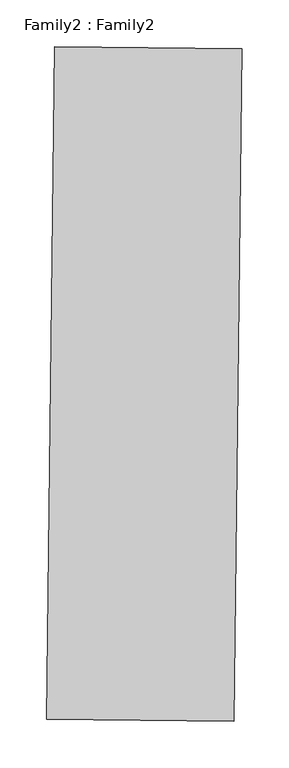
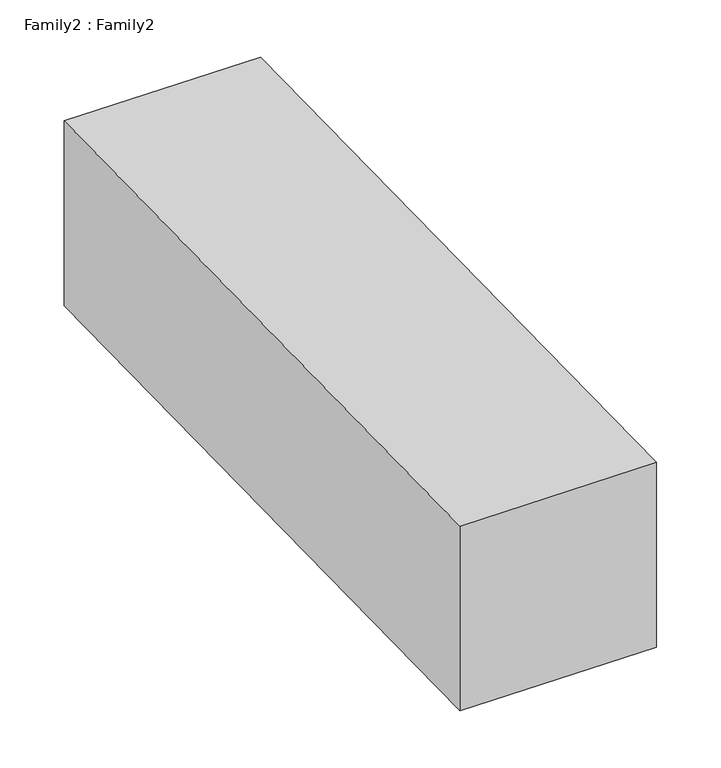
"""IFC4 building model written with IfcOpenShell, lengths in millimetres: proxy geometry, Family2 : Family2."""

from ifc_helpers import new_model, si_unit, origin, place, context, project, spatial, faceted_brep, source, transform, mapped, element, save


def family2_family2_c0c01265(model_context):
    return source(origin(), model_context, "Body", "Brep", [
        faceted_brep([(-3947.6024006, -6432.4470029, 1.0945136), (-3947.6024006, -6432.4470029, 201.0945136), (-3939.2403939, -5715.1531197, 202.060409), (-3939.2403939, -5715.1531197, 2.060409), (-3747.6112106, -6434.3242155, 201.0945136), (-3739.249204, -5717.0303324, 202.060409), (-3747.6112106, -6434.3242155, 1.0945136), (-3739.249204, -5717.0303324, 2.060409)], [[[0, 1, 2, 3]], [[1, 4, 5, 2]], [[4, 6, 7, 5]], [[6, 0, 3, 7]], [[3, 2, 5, 7]], [[0, 6, 4, 1]]]),
    ])


if __name__ == "__main__":
    model = new_model("IFC4")
    model_context = context("Model", 3, world=origin())
    ifc_project = project(units=[si_unit("LENGTHUNIT", "METRE", prefix="MILLI")], contexts=[model_context])
    site = spatial("IfcSite", under=ifc_project)
    building = spatial("IfcBuilding", under=site)
    placement = place(None, origin())
    family2_family2_shape = family2_family2_c0c01265(model_context)
    element("IfcBuildingElementProxy", 1, Name="Family2 : Family2", ObjectType="Family2 : Family2", at=placement, inside=building, context=model_context, shape_type="MappedRepresentation", body=[
        mapped(family2_family2_shape, transform((0.0, 0.0, 0.0), x_axis=(1.0, 0.0, 0.0), y_axis=(0.0, 1.0, 0.0), z_axis=(0.0, 0.0, 1.0))),
    ])
    save(model, "model.ifc")

# Revit data of these elements
# Type "Family2 : Family2"
#   Default Elevation = 0
